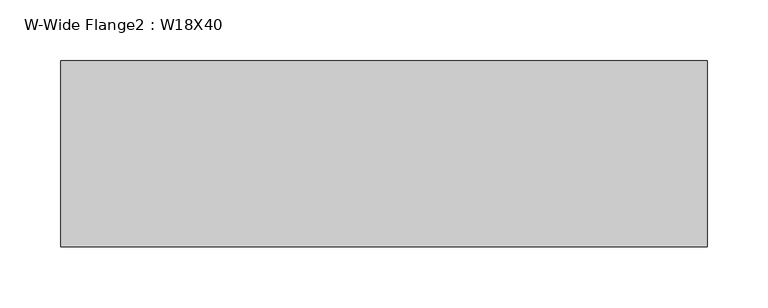
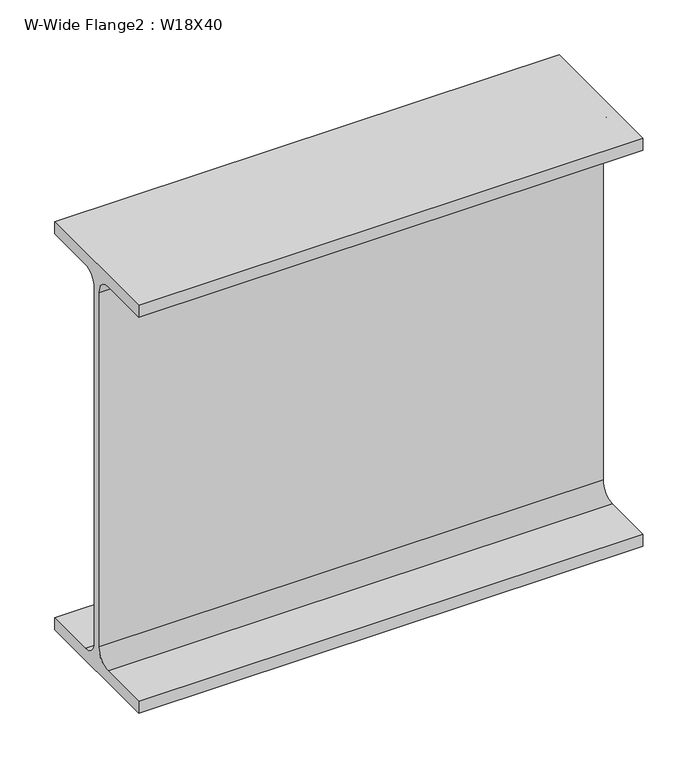
"""IFC4 building model written with IfcOpenShell, lengths in millimetres: beam geometry, W-Wide Flange2 : W18X40."""

from ifc_helpers import new_model, si_unit, point, frame, frame_2d, origin, place, context, project, spatial, polyline, circle_curve, trimmed, segment, composite_curve, outline, extrude, source, transform, mapped, element, save


def w_wide_flange2_w18x40_c53f6964(model_context):
    return source(origin(), model_context, "Body", "SweptSolid", [
        extrude(outline(composite_curve([segment(polyline([(76.454, -213.995), (76.454, -227.33), (-76.454, -227.33), (-76.454, -213.995), (-20.828, -213.995)]), True, "CONTINUOUS"), segment(trimmed(circle_curve(frame_2d((-20.828, -197.1675)), 16.8275), [point((-20.828, -213.995))], [point((-4.0005, -197.1675))], True, "CARTESIAN"), True, "CONTINUOUS"), segment(polyline([(-4.0005, -197.1675), (-4.0005, 197.1675)]), True, "CONTINUOUS"), segment(trimmed(circle_curve(frame_2d((-20.828, 197.1675)), 16.8275), [point((-4.0005, 197.1675))], [point((-20.828, 213.995))], True, "CARTESIAN"), True, "CONTINUOUS"), segment(polyline([(-20.828, 213.995), (-76.454, 213.995), (-76.454, 227.33), (76.454, 227.33), (76.454, 213.995), (20.828, 213.995)]), True, "CONTINUOUS"), segment(trimmed(circle_curve(frame_2d((20.828, 197.1675)), 16.8275), [point((20.828, 213.995))], [point((4.0005, 197.1675))], True, "CARTESIAN"), True, "CONTINUOUS"), segment(polyline([(4.0005, 197.1675), (4.0005, -197.1675)]), True, "CONTINUOUS"), segment(trimmed(circle_curve(frame_2d((20.828, -197.1675)), 16.8275), [point((4.0005, -197.1675))], [point((20.828, -213.995))], True, "CARTESIAN"), True, "CONTINUOUS"), segment(polyline([(20.828, -213.995), (76.454, -213.995)]), True, "CONTINUOUS")], self_intersect=False)), frame((-296.8625, 0.0, 0.0), z_axis=(1.0, 0.0, 0.0), x_axis=(0.0, 1.0, 0.0)), (0.0, 0.0, 1.0), 531.415625),
    ])


if __name__ == "__main__":
    model = new_model("IFC4")
    model_context = context("Model", 3, world=origin())
    ifc_project = project(units=[si_unit("LENGTHUNIT", "METRE", prefix="MILLI")], contexts=[model_context])
    site = spatial("IfcSite", under=ifc_project)
    building = spatial("IfcBuilding", under=site)
    placement = place(None, origin())
    w_wide_flange2_w18x40_shape = w_wide_flange2_w18x40_c53f6964(model_context)
    element("IfcBeam", 1, ObjectType="W-Wide Flange2 : W18X40", at=placement, inside=building, context=model_context, shape_type="MappedRepresentation", body=[
        mapped(w_wide_flange2_w18x40_shape, transform((0.0, 0.0, 0.0), x_axis=(1.0, 0.0, 0.0), y_axis=(0.0, 1.0, 0.0), z_axis=(0.0, 0.0, 1.0))),
    ])
    save(model, "model.ifc")

# Revit data of these elements
# Type "W-Wide Flange2 : W18X40"
#   Assembly Code = "B10"
#   W = 40
#   Length [instance default] = 5' - 0"
#   bf = 0' - 6.02"
#   d = 1' - 5.9"
#   k = 0' - 1 3/16"
#   k2 = 0' - 0.6625"
#   tf = 0' - 0.525"
#   tw = 0' - 0.315"
#   A = 0.0819444 SF
#   Structural Material [instance default] = Steel ASTM A992
# Element 1 (IfcBeam, "W-Wide Flange2 : W18X40")
#   Materials on its faces: "Steel ASTM A992"
# Materials
#   "Steel ASTM A992": class "Metal", colour RGB 199 199 199, transparency 0, Description = "Structural steel 50ksi", Cost = 0
